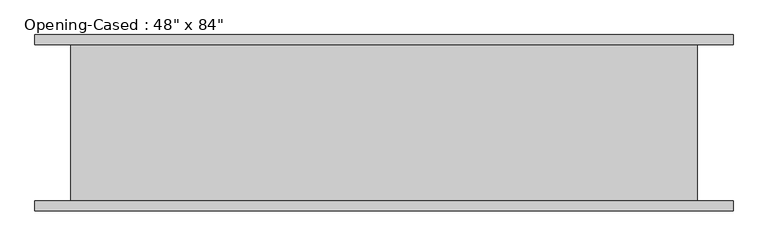
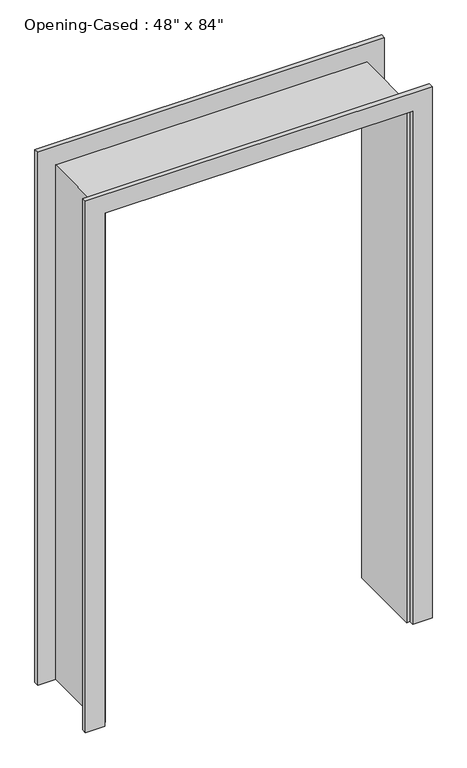
"""IFC4 building model written with IfcOpenShell, lengths in millimetres: proxy geometry."""

from ifc_helpers import new_model, si_unit, frame, origin, place, context, project, spatial, polyline, outline, extrude, faceted_brep, source, transform, mapped, element, save


def proxy_20ebd3de(model_context):
    return source(origin(), model_context, "Body", "SolidModel", [
        extrude(outline(polyline([(0.0, -611.4386567), (2127.25, -611.4386567), (2127.25, 595.0613433), (0.0, 595.0613433), (0.0, 671.2613433), (2203.45, 671.2613433), (2203.45, -687.6386567), (0.0, -687.6386567), (0.0, -611.4386567)])), frame((0.0, -171.45, 0.0), z_axis=(0.0, 1.0, 0.0), x_axis=(0.0, 0.0, 1.0)), (0.0, 0.0, 1.0), 19.05),
        extrude(outline(polyline([(0.0, 671.2613433), (2209.8, 671.2613433), (2209.8, -687.6386567), (0.0, -687.6386567), (0.0, -611.4386567), (2127.25, -611.4386567), (2127.25, 595.0613433), (0.0, 595.0613433), (0.0, 671.2613433)])), frame((0.0, 152.4, 0.0), z_axis=(0.0, 1.0, 0.0), x_axis=(0.0, 0.0, 1.0)), (0.0, 0.0, 1.0), 19.05),
        faceted_brep([(582.3613433, 152.4, 0.0), (601.4113433, 152.4, 0.0), (601.4113433, -152.4, 0.0), (582.3613433, -152.4, 0.0), (582.3613433, 152.4, 2114.55), (601.4113433, 152.4, 2133.6), (601.4113433, -152.4, 2133.6), (582.3613433, -152.4, 2114.55), (-598.7386567, 152.4, 2114.55), (-617.7886567, 152.4, 2133.6), (-617.7886567, -152.4, 2133.6), (-598.7386567, -152.4, 2114.55), (-598.7386567, 152.4, 0.0), (-598.7386567, -152.4, 0.0), (-617.7886567, -152.4, 0.0), (-617.7886567, 152.4, 0.0)], [[[0, 1, 2, 3]], [[1, 0, 4, 5]], [[2, 1, 5, 6]], [[3, 2, 6, 7]], [[0, 3, 7, 4]], [[5, 4, 8, 9]], [[6, 5, 9, 10]], [[7, 6, 10, 11]], [[4, 7, 11, 8]], [[12, 13, 14, 15]], [[9, 8, 12, 15]], [[10, 9, 15, 14]], [[11, 10, 14, 13]], [[8, 11, 13, 12]]]),
    ])


if __name__ == "__main__":
    model = new_model("IFC4")
    model_context = context("Model", 3, world=origin())
    ifc_project = project(units=[si_unit("LENGTHUNIT", "METRE", prefix="MILLI")], contexts=[model_context])
    site = spatial("IfcSite", under=ifc_project)
    building = spatial("IfcBuilding", under=site)
    placement = place(None, origin())
    proxy_shape = proxy_20ebd3de(model_context)
    element("IfcBuildingElementProxy", 1, Name="Opening-Cased : 48\" x 84\"", ObjectType="Opening-Cased : 48\" x 84\"", at=placement, inside=building, context=model_context, shape_type="MappedRepresentation", body=[
        mapped(proxy_shape, transform((0.0, 0.0, 0.0), x_axis=(1.0, 0.0, 0.0), y_axis=(0.0, 1.0, 0.0), z_axis=(0.0, 0.0, 1.0))),
    ])
    save(model, "model.ifc")

# Revit data of these elements
# Type "Opening-Cased : 48\" x 84\""
#   Height = 7' - 0"
#   Trim Thickness = 0' - 0 3/4"
#   Trim Width = 0' - 3"
#   Width = 4' - 0"
#   Frame Material = Door - Frame
#   Assembly Code = ""
# Element 1 (IfcBuildingElementProxy, "Opening-Cased : 48\" x 84\"")
#   Materials on its faces: "Door - Frame"
# Materials
#   "Door - Frame": class "Unassigned", colour RGB 118 70 51, transparency 0, Comments = "Rendering appearance not upgraded Rendering appearance not upgraded "
